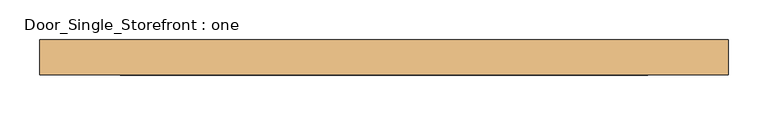
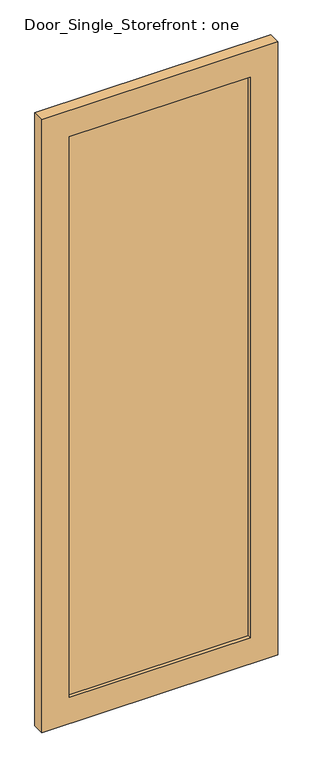
"""IFC4 building model written with IfcOpenShell, lengths in millimetres: door geometry, Door_Single_Storefront : one."""

from ifc_helpers import new_model, si_unit, frame, origin, place, context, project, spatial, polyline, outline, extrude, source, transform, mapped, element, save


def door_single_storefront_one_13bf0d0e(model_context):
    return source(origin(), model_context, "Body", "SweptSolid", [
        extrude(outline(polyline([(2387.6, -434.18125), (0.0, -434.18125), (0.0, 434.18125), (2387.6, 434.18125), (2387.6, -434.18125)]), holes=[polyline([(101.6, 332.58125), (101.6, -332.58125), (2286.0, -332.58125), (2286.0, 332.58125), (101.6, 332.58125)])]), frame((0.0, -19.05, 0.0), z_axis=(0.0, 1.0, 0.0), x_axis=(0.0, 0.0, 1.0)), (0.0, 0.0, 1.0), 44.45),
        extrude(outline(polyline([(332.58125, -6.35), (-332.58125, -6.35), (-332.58125, 12.7), (332.58125, 12.7), (332.58125, -6.35)])), frame((0.0, 0.0, 101.6), z_axis=(0.0, 0.0, 1.0), x_axis=(1.0, 0.0, 0.0)), (0.0, 0.0, 1.0), 2184.4),
    ])


if __name__ == "__main__":
    model = new_model("IFC4")
    model_context = context("Model", 3, world=origin())
    ifc_project = project(units=[si_unit("LENGTHUNIT", "METRE", prefix="MILLI")], contexts=[model_context])
    site = spatial("IfcSite", under=ifc_project)
    building = spatial("IfcBuilding", under=site)
    placement = place(None, origin())
    door_single_storefront_one_shape = door_single_storefront_one_13bf0d0e(model_context)
    element("IfcDoor", 1, ObjectType="Door_Single_Storefront : one", at=placement, inside=building, context=model_context, shape_type="MappedRepresentation", body=[
        mapped(door_single_storefront_one_shape, transform((0.0, 0.0, 0.0), x_axis=(1.0, 0.0, 0.0), y_axis=(0.0, 1.0, 0.0), z_axis=(0.0, 0.0, 1.0))),
    ])
    save(model, "model.ifc")

# Revit data of these elements
# Type "Door_Single_Storefront : one"
#   Type Mark = "27"
#   Analytic Construction = "<None>"
#   Stile_Width = 0' - 4"
#   Door_Thickness = 0' - 1 3/4"
#   Door_Offset = 0' - 1"
#   Glass_Material = Glass
#   Frame_Material = Aluminum
#   Function = (empty or 0)
# Element 1 (IfcDoor, "Door_Single_Storefront : one")
#   Materials on its faces: "Aluminum", "Glass"
# Materials
#   "Glass": class "Glass", colour RGB 142 168 196, transparency 0.75, Description = "Soda Lime Glass", Cost = 0
#   "Aluminum": class "Metal", colour RGB 226 226 226, transparency 0, Description = "Aluminum 6061", Cost = 0
